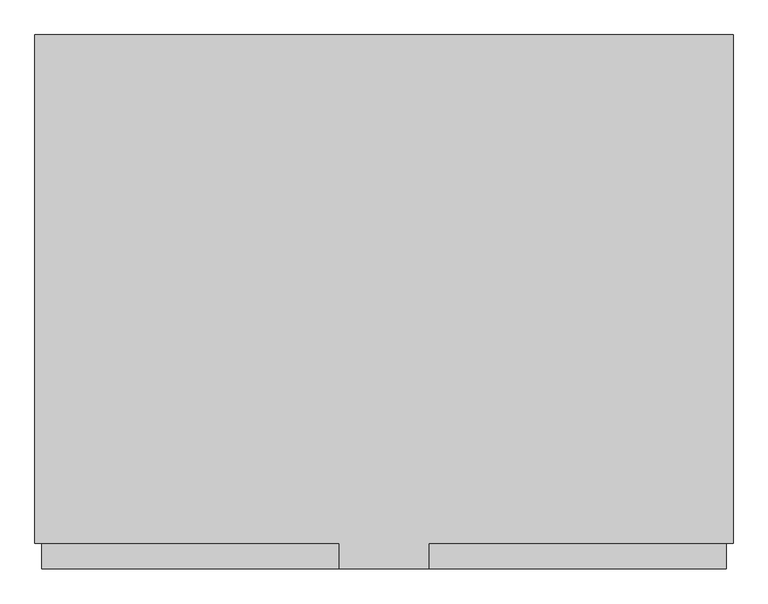
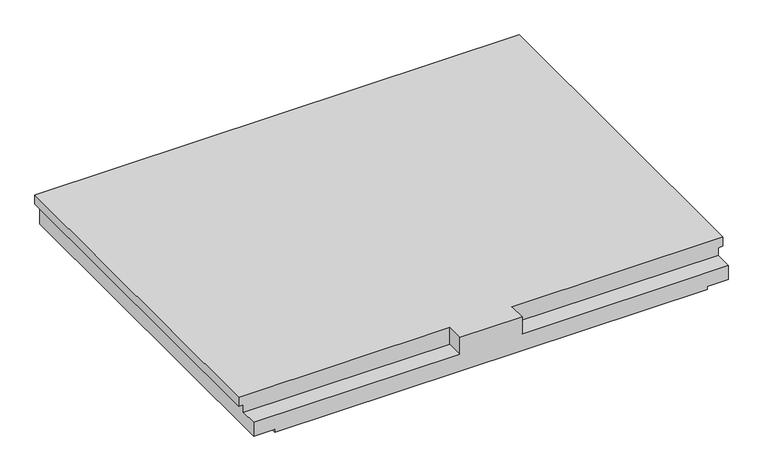
"""IFC4 building model written with IfcOpenShell, lengths in millimetres: proxy geometry, NLRS_24_GM_UN_rechthoekig bordes prefab-AV_gen_rsf : prefab bordes_gen__2300x3005."""

import ifcopenshell
import ifcopenshell.guid

model = None  # the IFC model being written
_history = None  # IfcOwnerHistory: only IFC2X3 demands one
_inside = {}  # id of a spatial element -> (the spatial element, [elements in it])
_under = {}  # id of a project, library or spatial element -> (it, [spatial elements below it])
_declared = {}  # id of a project -> (the project, [libraries it declares])
_typed = {}  # id of a type object -> (the type object, [elements of that type])
_made_of = {}  # id of a material, layer set ... -> (it, [elements and type objects made of it])


def new_model(schema):
    """Start an empty IFC model of exactly this schema.

    Asked for "IFC4X3", IfcOpenShell would pick the latest addendum, in which some entities
    have other attributes; the version numbers below select the first issue.
    IFC2X3 requires an IfcOwnerHistory on every rooted entity: one is made here for all.
    """
    global model, _history
    if schema == "IFC4X3":
        model = ifcopenshell.file(schema_version=(4, 3, 0, 0))
    else:
        model = ifcopenshell.file(schema=schema)
    _inside.clear()
    _under.clear()
    _declared.clear()
    _typed.clear()
    _made_of.clear()
    _history = None
    if model.schema == "IFC2X3":
        org = make("IfcOrganization", Name="unknown")
        user = make(
            "IfcPersonAndOrganization",
            ThePerson=make("IfcPerson", FamilyName="unknown"),
            TheOrganization=org,
        )
        app = make(
            "IfcApplication",
            ApplicationDeveloper=org,
            Version="unknown",
            ApplicationFullName="unknown",
            ApplicationIdentifier="unknown",
        )
        _history = make(
            "IfcOwnerHistory",
            OwningUser=user,
            OwningApplication=app,
            ChangeAction="ADDED",
            CreationDate=0,
        )
    return model


def make(cls, **values):
    """One entity of the class cls with the attributes given. An attribute that is None is left unset."""
    return model.create_entity(
        cls, **{name: value for name, value in values.items() if value is not None}
    )


def rooted(cls, **values):
    """An entity with a GlobalId (a new one), such as an element, a storey or a relation."""
    return make(cls, GlobalId=ifcopenshell.guid.new(), OwnerHistory=_history, **values)


def si_unit(unit_type, name, prefix=None):
    """IfcSIUnit, for example si_unit("LENGTHUNIT", "METRE", prefix="MILLI")."""
    return make("IfcSIUnit", UnitType=unit_type, Prefix=prefix, Name=name)


def assignment(units):
    """IfcUnitAssignment: the units of a project."""
    return None if units is None else make("IfcUnitAssignment", Units=units)


def point(xyz):
    """IfcCartesianPoint."""
    return None if xyz is None else make("IfcCartesianPoint", Coordinates=xyz)


def direction(xyz):
    """IfcDirection."""
    return None if xyz is None else make("IfcDirection", DirectionRatios=xyz)


def frame(location, z_axis=None, x_axis=None):
    """IfcAxis2Placement3D, a coordinate frame: its origin and axes. An axis left out is left unset."""
    return make(
        "IfcAxis2Placement3D",
        Location=point(location),
        Axis=direction(z_axis),
        RefDirection=direction(x_axis),
    )


def origin():
    """The frame at (0, 0, 0) with its axes left unset."""
    return frame((0.0, 0.0, 0.0))


def place(relative_to, where):
    """IfcLocalPlacement: puts the frame where relative to a parent placement (None: the world)."""
    return make(
        "IfcLocalPlacement", PlacementRelTo=relative_to, RelativePlacement=where
    )


def context(
    kind, dimensions, precision=None, world=None, true_north=None, identifier=None
):
    """IfcGeometricRepresentationContext, for example the 3D "Model" context."""
    return make(
        "IfcGeometricRepresentationContext",
        ContextIdentifier=identifier,
        ContextType=kind,
        CoordinateSpaceDimension=dimensions,
        Precision=precision,
        WorldCoordinateSystem=world,
        TrueNorth=true_north,
    )


def project(units=None, contexts=None):
    """IfcProject with its units and contexts."""
    return rooted(
        "IfcProject",
        Name="project",
        RepresentationContexts=contexts,
        UnitsInContext=assignment(units),
    )


def spatial(cls, under=None, at=None, **own):
    """A site, building, storey or space (cls), placed at a placement, below another one or the project."""
    s = rooted(cls, ObjectPlacement=at, **own)
    if under is not None:
        _under.setdefault(under.id(), (under, []))[1].append(s)
    return s


def faces_of(points, faces, orient=None, outer=None):
    """IfcFace entities. A face is a list of loops; a loop is a list of indices into points, from 0.

    orient and outer hold one flag for each loop. By default every Orientation is true, the
    first loop of a face is its IfcFaceOuterBound and the others are IfcFaceBound.
    """
    made = []
    for i, loops in enumerate(faces):
        bounds = []
        for j, loop in enumerate(loops):
            is_outer = j == 0 if outer is None else outer[i][j]
            bounds.append(
                make(
                    "IfcFaceOuterBound" if is_outer else "IfcFaceBound",
                    Bound=make("IfcPolyLoop", Polygon=[points[k] for k in loop]),
                    Orientation=True if orient is None else orient[i][j],
                )
            )
        made.append(make("IfcFace", Bounds=bounds))
    return made


def faceted_brep(points, faces, orient=None, outer=None, voids=None):
    """IfcFacetedBrep: a solid bounded by flat faces; with voids (closed shells), ...WithVoids."""
    shared = [point(p) for p in points]
    hull = make("IfcClosedShell", CfsFaces=faces_of(shared, faces, orient, outer))
    if voids is None:
        return make("IfcFacetedBrep", Outer=hull)
    return make(
        "IfcFacetedBrepWithVoids",
        Outer=hull,
        Voids=[
            make(cls, CfsFaces=faces_of(shared, fs, o, b)) for cls, fs, o, b in voids
        ],
    )


def shape(context_of_items, identifier, shape_type, items):
    """IfcShapeRepresentation: the items that make up one representation, for example the "Body"."""
    return make(
        "IfcShapeRepresentation",
        ContextOfItems=context_of_items,
        RepresentationIdentifier=identifier,
        RepresentationType=shape_type,
        Items=items,
    )


def source(mapping_origin, context_of_items, identifier, shape_type, items):
    """IfcRepresentationMap: a shape defined once, which mapped items show again and again."""
    return make(
        "IfcRepresentationMap",
        MappingOrigin=mapping_origin,
        MappedRepresentation=shape(context_of_items, identifier, shape_type, items),
    )


def transform(
    local_origin,
    x_axis=None,
    y_axis=None,
    z_axis=None,
    scale=None,
    scale2=None,
    scale3=None,
    uniform=True,
):
    """IfcCartesianTransformationOperator3D, or its non-uniform kind. x_axis, y_axis, z_axis: its Axis1, 2, 3."""
    if uniform:
        return make(
            "IfcCartesianTransformationOperator3D",
            Axis1=direction(x_axis),
            Axis2=direction(y_axis),
            LocalOrigin=point(local_origin),
            Scale=scale,
            Axis3=direction(z_axis),
        )
    return make(
        "IfcCartesianTransformationOperator3DnonUniform",
        Axis1=direction(x_axis),
        Axis2=direction(y_axis),
        LocalOrigin=point(local_origin),
        Scale=scale,
        Axis3=direction(z_axis),
        Scale2=scale2,
        Scale3=scale3,
    )


def mapped(mapping_source, mapping_target):
    """IfcMappedItem: shows the shape of a source again, moved by a transform."""
    return make(
        "IfcMappedItem", MappingSource=mapping_source, MappingTarget=mapping_target
    )


def made_of(thing, what):
    """Note that an element or type object is made of a material, layer set ...; save() writes the relation."""
    if what is not None:
        _made_of.setdefault(what.id(), (what, []))[1].append(thing)
    return thing


def element(
    cls,
    number,
    at=None,
    inside=None,
    cuts=None,
    type_object=None,
    material=None,
    context=None,
    identifier="Body",
    shape_type=None,
    held_by="IfcProductDefinitionShape",
    body=None,
    shapes=None,
    **own,
):
    """One element of the class cls, such as IfcWall. Its Tag is "e" and its number.

    at: its placement. inside: the storey or other place that contains it. cuts: it is an
    opening in that element (IfcRelVoidsElement). A single representation is given by context,
    identifier, shape_type and body (its items); several are given by shapes. held_by: the class
    of the entity that holds the representations. save() writes the other relations.
    """
    e = rooted(cls, Tag="e%d" % number, ObjectPlacement=at, **own)
    if body is not None:
        shapes = [shape(context, identifier, shape_type, body)]
    if shapes is not None:
        e.Representation = make(held_by, Representations=shapes)
    if inside is not None:
        _inside.setdefault(inside.id(), (inside, []))[1].append(e)
    if cuts is not None:
        rooted(
            "IfcRelVoidsElement", RelatingBuildingElement=cuts, RelatedOpeningElement=e
        )
    if type_object is not None:
        _typed.setdefault(type_object.id(), (type_object, []))[1].append(e)
    return made_of(e, material)


def aggregate(whole, parts):
    """IfcRelAggregates: a whole, such as a stair, and the parts it consists of."""
    return rooted("IfcRelAggregates", RelatingObject=whole, RelatedObjects=parts)


def save(model, path):
    """Write the relations noted so far, then the file.

    IfcRelAggregates (storeys below a building ...), IfcRelContainedInSpatialStructure (elements
    in a storey), IfcRelDefinesByType, IfcRelAssociatesMaterial and IfcRelDeclares: one each for
    every whole, place, type object, material and project.
    """
    for whole, parts in _under.values():
        aggregate(whole, parts)
    for where, things in _inside.values():
        rooted(
            "IfcRelContainedInSpatialStructure",
            RelatedElements=things,
            RelatingStructure=where,
        )
    for kind, things in _typed.values():
        rooted("IfcRelDefinesByType", RelatedObjects=things, RelatingType=kind)
    for what, things in _made_of.values():
        rooted("IfcRelAssociatesMaterial", RelatedObjects=things, RelatingMaterial=what)
    for by, libraries in _declared.values():
        rooted("IfcRelDeclares", RelatingContext=by, RelatedDefinitions=libraries)
    model.write(path)


def generic_models_8b033359(model_context):
    return source(origin(), model_context, "Body", "Brep", [
        faceted_brep([(1502.5, -2190.0, 0.0), (1502.5, -2190.0, -60.0), (1502.5, 0.0, -60.0), (1502.5, 0.0, 0.0), (192.5, -2300.0, -110.0), (1472.5, -2300.0, -110.0), (1472.5, -2190.0, -110.0), (192.5, -2190.0, -110.0), (192.5, -2190.0, 0.0), (1472.5, -2190.0, -60.0), (192.5, -2300.0, 0.0), (-192.5, -2300.0, 0.0), (-192.5, -2190.0, 0.0), (-192.5, -2190.0, -110.0), (-192.5, -2300.0, -110.0), (-1502.5, 0.0, 0.0), (-1502.5, 0.0, -60.0), (-1502.5, -2190.0, -60.0), (-1502.5, -2190.0, 0.0), (-1472.5, -2300.0, -110.0), (-1472.5, -2300.0, -200.0), (-1342.5, -2300.0, -200.0), (-1342.5, -2300.0, -220.0), (1342.5, -2300.0, -220.0), (1342.5, -2300.0, -200.0), (1472.5, -2300.0, -200.0), (-1472.5, -2190.0, -110.0), (-1472.5, -2190.0, -60.0), (1472.5, 0.0, -60.0), (1472.5, 0.0, -200.0), (1342.5, 0.0, -200.0), (1342.5, 0.0, -220.0), (-1342.5, 0.0, -220.0), (-1342.5, 0.0, -200.0), (-1472.5, 0.0, -200.0), (-1472.5, 0.0, -60.0)], [[[0, 1, 2, 3]], [[4, 5, 6, 7]], [[8, 7, 6, 9, 1, 0]], [[10, 4, 7, 8]], [[11, 12, 13, 14]], [[15, 16, 17, 18]], [[19, 20, 21, 22, 23, 24, 25, 5, 4, 10, 11, 14]], [[14, 13, 26, 19]], [[18, 17, 27, 26, 13, 12]], [[18, 12, 11, 10, 8, 0, 3, 15]], [[15, 3, 2, 28, 29, 30, 31, 32, 33, 34, 35, 16]], [[32, 31, 23, 22]], [[27, 17, 16, 35]], [[20, 19, 26, 27, 35, 34]], [[34, 33, 21, 20]], [[33, 32, 22, 21]], [[28, 2, 1, 9]], [[29, 28, 9, 6, 5, 25]], [[25, 24, 30, 29]], [[24, 23, 31, 30]]]),
    ])


if __name__ == "__main__":
    model = new_model("IFC4")
    model_context = context("Model", 3, world=origin())
    ifc_project = project(units=[si_unit("LENGTHUNIT", "METRE", prefix="MILLI")], contexts=[model_context])
    site = spatial("IfcSite", under=ifc_project)
    building = spatial("IfcBuilding", under=site)
    placement = place(None, origin())
    generic_models_shape = generic_models_8b033359(model_context)
    element("IfcBuildingElementProxy", 1, Name="NLRS_24_GM_UN_rechthoekig bordes prefab-AV_gen_rsf : prefab bordes_gen__2300x3005", ObjectType="NLRS_24_GM_UN_rechthoekig bordes prefab-AV_gen_rsf : prefab bordes_gen__2300x3005", at=placement, inside=building, context=model_context, shape_type="MappedRepresentation", body=[
        mapped(generic_models_shape, transform((0.0, 0.0, 0.0), x_axis=(1.0, 0.0, 0.0), y_axis=(0.0, 1.0, 0.0), z_axis=(0.0, 0.0, 1.0))),
    ])
    save(model, "model.ifc")

# Revit data of these elements
# Type "NLRS_24_GM_UN_rechthoekig bordes prefab-AV_gen_rsf : prefab bordes_gen__2300x3005"
#   Export Type to IFC As = "IfcStair"
#   Type IfcGUID = "2CEqVLPNH8KRN7ghwV3abv"
#   Type Comments = " "
#   Model = " "
#   Manufacturer = " "
#   Description = "rechthoekig bordes prefab\r\n1930x4395"
#   Assembly Code = "24.15"
#   Width = 3005 mm
#   Thickness = 220 mm
#   Perimeter = 10610 mm
#   NLRS_C_lengte_02 = 1310 mm
#   NLRS_C_lengte_01 = 1310 mm
#   NLRS_C_hoogte_02 = 110 mm
#   NLRS_C_hoogte_01 = 110 mm
#   NLRS_C_diepte_04 = 2300 mm
#   NLRS_C_diepte_03 = 2300 mm
#   NLRS_C_diepte_02 = 110 mm
#   NLRS_C_diepte_01 = 110 mm
#   Length = 2300 mm
#   Default Elevation = 1219.2 mm
#   Area = 6.9115 m²
#   NLRS_C_materiaal = NLRS_f2_beton prefab_gen_rsf
#   Keynote = ""
# Element 1 (IfcBuildingElementProxy, "NLRS_24_GM_UN_rechthoekig bordes prefab-AV_gen_rsf : prefab bordes_gen__2300x3005")
#   Materials on its faces: "NLRS_f2_beton prefab_gen_rsf"
# Materials
#   "NLRS_f2_beton prefab_gen_rsf": class "F - Niet gebakken kunststeen", colour RGB 129 133 118, transparency 0, Keynote = "f2", Manufacturer = "Revit Standards Foundation", URL = "www.revitstandards.org", Description = "beton prefab", Cost = 0
